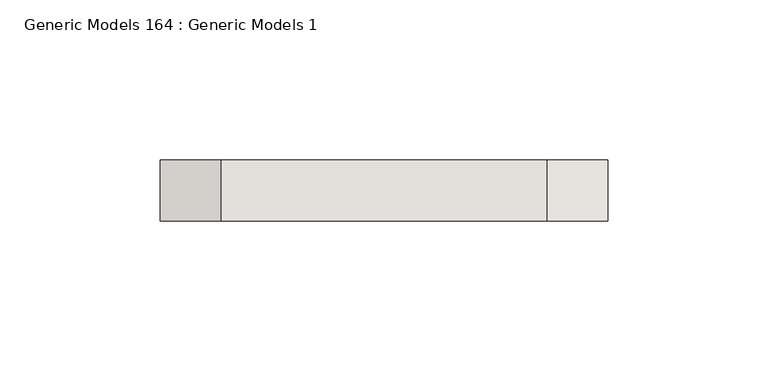
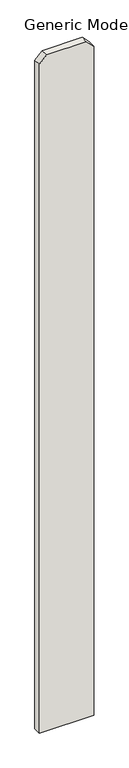
"""IFC4 building model written with IfcOpenShell, lengths in millimetres: wall geometry, Generic Models 164 : Generic Models 1."""

from ifc_helpers import new_model, si_unit, frame, origin, place, context, project, spatial, polyline, outline, extrude, source, transform, mapped, element, save


def generic_models_164_generic_models_1_0a78b959(model_context):
    return source(origin(), model_context, "Body", "SweptSolid", [
        extrude(outline(polyline([(76.2, 323975.4125), (1885.95, 323975.4125), (1905.0, 323956.3625), (1905.0, 323854.7625), (1885.95, 323835.7125), (76.2, 323835.7125), (76.2, 323975.4125)])), frame((0.0, 547.6875, 0.0), z_axis=(0.0, 1.0, 0.0), x_axis=(0.0, 0.0, 1.0)), (0.0, 0.0, 1.0), 19.05),
    ])


if __name__ == "__main__":
    model = new_model("IFC4")
    model_context = context("Model", 3, world=origin())
    ifc_project = project(units=[si_unit("LENGTHUNIT", "METRE", prefix="MILLI")], contexts=[model_context])
    site = spatial("IfcSite", under=ifc_project)
    building = spatial("IfcBuilding", under=site)
    placement = place(None, origin())
    generic_models_164_generic_models_1_shape = generic_models_164_generic_models_1_0a78b959(model_context)
    element("IfcWall", 1, ObjectType="Generic Models 164 : Generic Models 1", at=placement, inside=building, context=model_context, shape_type="MappedRepresentation", body=[
        mapped(generic_models_164_generic_models_1_shape, transform((0.0, 0.0, 0.0), x_axis=(1.0, 0.0, 0.0), y_axis=(0.0, 1.0, 0.0), z_axis=(0.0, 0.0, 1.0))),
    ])
    save(model, "model.ifc")

# Revit data of these elements
# Element 1 (IfcWall, "Generic Models 164 : Generic Models 1")
#   Materials on its faces: "VERTICAL 1X6 CEDAR PLANKS W/ CLEAR WOOD SEALER"
# Materials
#   "VERTICAL 1X6 CEDAR PLANKS W/ CLEAR WOOD SEALER": class "Wood", colour RGB 234 198 147, transparency 0, Description = "Pinus Echinata", Cost = 0
